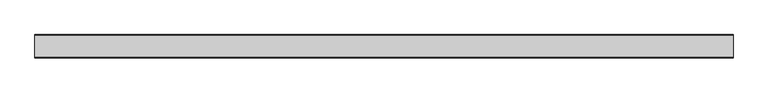
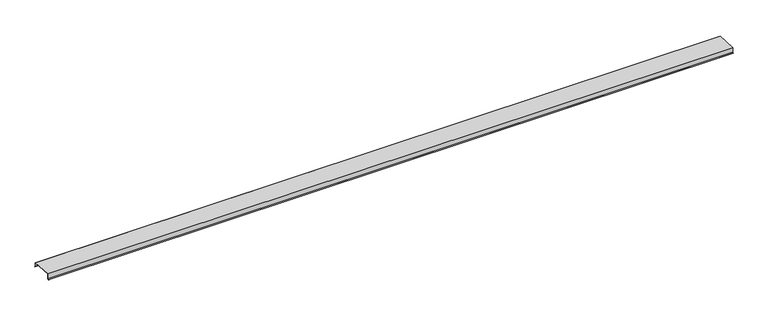
"""IFC4 building model written with IfcOpenShell, lengths in millimetres: proxy geometry, Generic Models 7:Generic Models 1:5:Generic Models 1:5 : Generic Models 7:Generic Models 1:337419:7 : Generic Models 7:Generic Models 1:5:Generic Models 1:5 : Generic Models 7:Generic Models 1:337419:311462."""

from ifc_helpers import new_model, si_unit, frame, origin, place, context, project, spatial, polyline, outline, extrude, source, transform, mapped, element, save


def generic_models_cf842490(model_context):
    return source(origin(), model_context, "Body", "SweptSolid", [
        extrude(outline(polyline([(-579111.8163841, 6099.8348677), (-579111.8163841, 6188.1524863), (-578729.2288841, 6168.101925), (-578729.2288841, 6099.8348677), (-578716.5288841, 6087.1348677), (-578717.6514161, 6086.0123357), (-578730.8163841, 6099.1773037), (-578730.8163841, 6166.5954438), (-579110.2288841, 6186.4796103), (-579110.2288841, 6099.1773037), (-579123.3938521, 6086.0123357), (-579124.5163841, 6087.1348677), (-579111.8163841, 6099.8348677)])), frame((560646.6492239, 0.0, 0.0), z_axis=(1.0, 0.0, 0.0), x_axis=(0.0, 1.0, 0.0)), (0.0, 0.0, 1.0), 12250.7375001),
    ])


if __name__ == "__main__":
    model = new_model("IFC4")
    model_context = context("Model", 3, world=origin())
    ifc_project = project(units=[si_unit("LENGTHUNIT", "METRE", prefix="MILLI")], contexts=[model_context])
    site = spatial("IfcSite", under=ifc_project)
    building = spatial("IfcBuilding", under=site)
    placement = place(None, origin())
    generic_models_shape = generic_models_cf842490(model_context)
    element("IfcBuildingElementProxy", 1, Name="Generic Models 7:Generic Models 1:5:Generic Models 1:5 : Generic Models 7:Generic Models 1:337419:7 : Generic Models 7:Generic Models 1:5:Generic Models 1:5 : Generic Models 7:Generic Models 1:337419:311462", ObjectType="Generic Models 7:Generic Models 1:5:Generic Models 1:5 : Generic Models 7:Generic Models 1:337419:7 : Generic Models 7:Generic Models 1:5:Generic Models 1:5 : Generic Models 7:Generic Models 1:337419:311462", at=placement, inside=building, context=model_context, shape_type="MappedRepresentation", body=[
        mapped(generic_models_shape, transform((0.0, 0.0, 0.0), x_axis=(1.0, 0.0, 0.0), y_axis=(0.0, 1.0, 0.0), z_axis=(0.0, 0.0, 1.0))),
    ])
    save(model, "model.ifc")

# Revit data of these elements
# Type "Generic Models 7:Generic Models 1:5:Generic Models 1:5 : Generic Models 7:Generic Models 1:337419:7 : Generic Models 7:Generic Models 1:5:Generic Models 1:5 : Generic Models 7:Generic Models 1:337419:311462"
#   NameOverride = "Generic Models 7:Generic Models 1:5:Generic Models 1:5 : Generic Models 7:Generic Models 1:337419:311462"
#   ObjectTypeOverride = "Generic Models 1:5 : Generic Models 7:Generic Models 1:337419"
#   Reference = "Generic Models 1"
#   Tag = "311462"
# Element 1 (IfcBuildingElementProxy, "Generic Models 7:Generic Models 1:5:Generic Models 1:5 : Generic Models 7:Generic Models 1:337419:7 : Generic Models 7:Generic Models 1:5:Generic Models 1:5 : Generic Models 7:Generic Models 1:337419:311462")
#   Materials on its faces: "SHEET METAL COPING (COLOR TO MATCH RESIN PANEL)"
# Materials
#   "SHEET METAL COPING (COLOR TO MATCH RESIN PANEL)": class "Generic", colour RGB 240 240 240, transparency 0, Keynote = "M07711300.01", Cost = 0
